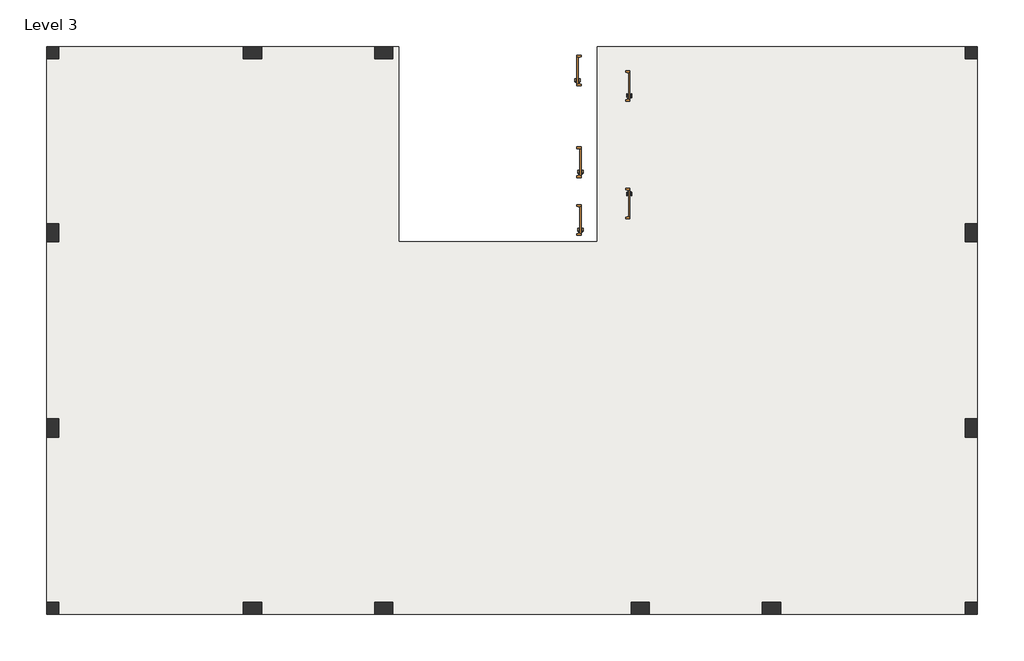
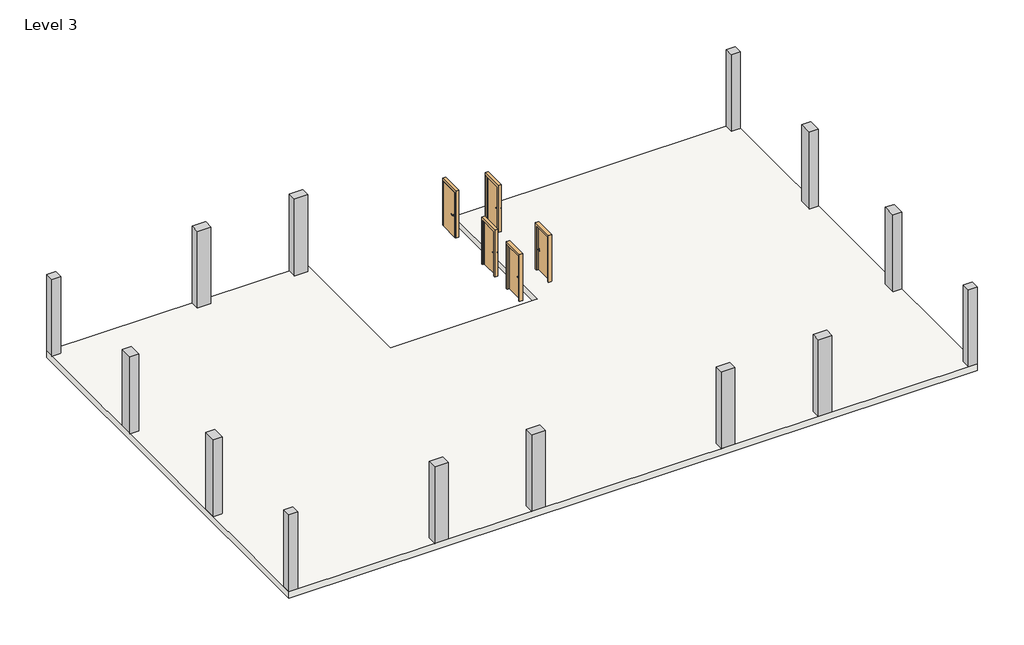
# One storey: 14 columns, 5 doors, 1 slab.
"""IFC4 building model written with IfcOpenShell, lengths in millimetres."""

import ifcopenshell
import ifcopenshell.guid

model = None  # the IFC model being written
_history = None  # IfcOwnerHistory: only IFC2X3 demands one
_inside = {}  # id of a spatial element -> (the spatial element, [elements in it])
_under = {}  # id of a project, library or spatial element -> (it, [spatial elements below it])
_declared = {}  # id of a project -> (the project, [libraries it declares])
_typed = {}  # id of a type object -> (the type object, [elements of that type])
_made_of = {}  # id of a material, layer set ... -> (it, [elements and type objects made of it])


def new_model(schema):
    """Start an empty IFC model of exactly this schema.

    Asked for "IFC4X3", IfcOpenShell would pick the latest addendum, in which some entities
    have other attributes; the version numbers below select the first issue.
    IFC2X3 requires an IfcOwnerHistory on every rooted entity: one is made here for all.
    """
    global model, _history
    if schema == "IFC4X3":
        model = ifcopenshell.file(schema_version=(4, 3, 0, 0))
    else:
        model = ifcopenshell.file(schema=schema)
    _inside.clear()
    _under.clear()
    _declared.clear()
    _typed.clear()
    _made_of.clear()
    _history = None
    if model.schema == "IFC2X3":
        org = make("IfcOrganization", Name="unknown")
        user = make(
            "IfcPersonAndOrganization",
            ThePerson=make("IfcPerson", FamilyName="unknown"),
            TheOrganization=org,
        )
        app = make(
            "IfcApplication",
            ApplicationDeveloper=org,
            Version="unknown",
            ApplicationFullName="unknown",
            ApplicationIdentifier="unknown",
        )
        _history = make(
            "IfcOwnerHistory",
            OwningUser=user,
            OwningApplication=app,
            ChangeAction="ADDED",
            CreationDate=0,
        )
    return model


def make(cls, **values):
    """One entity of the class cls with the attributes given. An attribute that is None is left unset."""
    return model.create_entity(
        cls, **{name: value for name, value in values.items() if value is not None}
    )


def rooted(cls, **values):
    """An entity with a GlobalId (a new one), such as an element, a storey or a relation."""
    return make(cls, GlobalId=ifcopenshell.guid.new(), OwnerHistory=_history, **values)


def si_unit(unit_type, name, prefix=None):
    """IfcSIUnit, for example si_unit("LENGTHUNIT", "METRE", prefix="MILLI")."""
    return make("IfcSIUnit", UnitType=unit_type, Prefix=prefix, Name=name)


def assignment(units):
    """IfcUnitAssignment: the units of a project."""
    return None if units is None else make("IfcUnitAssignment", Units=units)


def point(xyz):
    """IfcCartesianPoint."""
    return None if xyz is None else make("IfcCartesianPoint", Coordinates=xyz)


def direction(xyz):
    """IfcDirection."""
    return None if xyz is None else make("IfcDirection", DirectionRatios=xyz)


def frame(location, z_axis=None, x_axis=None):
    """IfcAxis2Placement3D, a coordinate frame: its origin and axes. An axis left out is left unset."""
    return make(
        "IfcAxis2Placement3D",
        Location=point(location),
        Axis=direction(z_axis),
        RefDirection=direction(x_axis),
    )


def frame_2d(location, x_axis=None):
    """IfcAxis2Placement2D, a coordinate frame in the plane: its origin and x axis."""
    return make(
        "IfcAxis2Placement2D", Location=point(location), RefDirection=direction(x_axis)
    )


def origin():
    """The frame at (0, 0, 0) with its axes left unset."""
    return frame((0.0, 0.0, 0.0))


def origin_with_axes():
    """The frame at (0, 0, 0) with the z axis (0, 0, 1) and the x axis (1, 0, 0) written out."""
    return frame((0.0, 0.0, 0.0), z_axis=(0.0, 0.0, 1.0), x_axis=(1.0, 0.0, 0.0))


def place(relative_to, where):
    """IfcLocalPlacement: puts the frame where relative to a parent placement (None: the world)."""
    return make(
        "IfcLocalPlacement", PlacementRelTo=relative_to, RelativePlacement=where
    )


def context(
    kind, dimensions, precision=None, world=None, true_north=None, identifier=None
):
    """IfcGeometricRepresentationContext, for example the 3D "Model" context."""
    return make(
        "IfcGeometricRepresentationContext",
        ContextIdentifier=identifier,
        ContextType=kind,
        CoordinateSpaceDimension=dimensions,
        Precision=precision,
        WorldCoordinateSystem=world,
        TrueNorth=true_north,
    )


def project(units=None, contexts=None):
    """IfcProject with its units and contexts."""
    return rooted(
        "IfcProject",
        Name="project",
        RepresentationContexts=contexts,
        UnitsInContext=assignment(units),
    )


def spatial(cls, under=None, at=None, **own):
    """A site, building, storey or space (cls), placed at a placement, below another one or the project."""
    s = rooted(cls, ObjectPlacement=at, **own)
    if under is not None:
        _under.setdefault(under.id(), (under, []))[1].append(s)
    return s


def polyline(points):
    """IfcPolyline through the points."""
    return make("IfcPolyline", Points=[point(p) for p in points])


def circle_curve(where, radius):
    """IfcCircle in the frame where."""
    return make("IfcCircle", Position=where, Radius=radius)


def ellipse_curve(where, semi_axis1, semi_axis2):
    """IfcEllipse in the frame where."""
    return make(
        "IfcEllipse", Position=where, SemiAxis1=semi_axis1, SemiAxis2=semi_axis2
    )


def trimmed(basis, trim1, trim2, sense, master):
    """IfcTrimmedCurve: the piece of a basis curve between two trims."""
    return make(
        "IfcTrimmedCurve",
        BasisCurve=basis,
        Trim1=trim1,
        Trim2=trim2,
        SenseAgreement=sense,
        MasterRepresentation=master,
    )


def segment(curve, same_sense, transition):
    """IfcCompositeCurveSegment."""
    return make(
        "IfcCompositeCurveSegment",
        Transition=transition,
        SameSense=same_sense,
        ParentCurve=curve,
    )


def composite_curve(segments, self_intersect=None):
    """IfcCompositeCurve: segments joined end to end."""
    return make("IfcCompositeCurve", Segments=segments, SelfIntersect=self_intersect)


def outline(outer, holes=None, kind="AREA"):
    """IfcArbitraryClosedProfileDef: a profile drawn as a closed curve; with holes, ...WithVoids."""
    if holes is None:
        return make("IfcArbitraryClosedProfileDef", ProfileType=kind, OuterCurve=outer)
    return make(
        "IfcArbitraryProfileDefWithVoids",
        ProfileType=kind,
        OuterCurve=outer,
        InnerCurves=holes,
    )


def extrude(swept, where, along, depth):
    """IfcExtrudedAreaSolid: the profile swept, set in the frame where, extruded along a direction by depth."""
    return make(
        "IfcExtrudedAreaSolid",
        SweptArea=swept,
        Position=where,
        ExtrudedDirection=direction(along),
        Depth=depth,
    )


def faces_of(points, faces, orient=None, outer=None):
    """IfcFace entities. A face is a list of loops; a loop is a list of indices into points, from 0.

    orient and outer hold one flag for each loop. By default every Orientation is true, the
    first loop of a face is its IfcFaceOuterBound and the others are IfcFaceBound.
    """
    made = []
    for i, loops in enumerate(faces):
        bounds = []
        for j, loop in enumerate(loops):
            is_outer = j == 0 if outer is None else outer[i][j]
            bounds.append(
                make(
                    "IfcFaceOuterBound" if is_outer else "IfcFaceBound",
                    Bound=make("IfcPolyLoop", Polygon=[points[k] for k in loop]),
                    Orientation=True if orient is None else orient[i][j],
                )
            )
        made.append(make("IfcFace", Bounds=bounds))
    return made


def faceted_brep(points, faces, orient=None, outer=None, voids=None):
    """IfcFacetedBrep: a solid bounded by flat faces; with voids (closed shells), ...WithVoids."""
    shared = [point(p) for p in points]
    hull = make("IfcClosedShell", CfsFaces=faces_of(shared, faces, orient, outer))
    if voids is None:
        return make("IfcFacetedBrep", Outer=hull)
    return make(
        "IfcFacetedBrepWithVoids",
        Outer=hull,
        Voids=[
            make(cls, CfsFaces=faces_of(shared, fs, o, b)) for cls, fs, o, b in voids
        ],
    )


def shape(context_of_items, identifier, shape_type, items):
    """IfcShapeRepresentation: the items that make up one representation, for example the "Body"."""
    return make(
        "IfcShapeRepresentation",
        ContextOfItems=context_of_items,
        RepresentationIdentifier=identifier,
        RepresentationType=shape_type,
        Items=items,
    )


def source(mapping_origin, context_of_items, identifier, shape_type, items):
    """IfcRepresentationMap: a shape defined once, which mapped items show again and again."""
    return make(
        "IfcRepresentationMap",
        MappingOrigin=mapping_origin,
        MappedRepresentation=shape(context_of_items, identifier, shape_type, items),
    )


def transform(
    local_origin,
    x_axis=None,
    y_axis=None,
    z_axis=None,
    scale=None,
    scale2=None,
    scale3=None,
    uniform=True,
):
    """IfcCartesianTransformationOperator3D, or its non-uniform kind. x_axis, y_axis, z_axis: its Axis1, 2, 3."""
    if uniform:
        return make(
            "IfcCartesianTransformationOperator3D",
            Axis1=direction(x_axis),
            Axis2=direction(y_axis),
            LocalOrigin=point(local_origin),
            Scale=scale,
            Axis3=direction(z_axis),
        )
    return make(
        "IfcCartesianTransformationOperator3DnonUniform",
        Axis1=direction(x_axis),
        Axis2=direction(y_axis),
        LocalOrigin=point(local_origin),
        Scale=scale,
        Axis3=direction(z_axis),
        Scale2=scale2,
        Scale3=scale3,
    )


def mapped(mapping_source, mapping_target):
    """IfcMappedItem: shows the shape of a source again, moved by a transform."""
    return make(
        "IfcMappedItem", MappingSource=mapping_source, MappingTarget=mapping_target
    )


def made_of(thing, what):
    """Note that an element or type object is made of a material, layer set ...; save() writes the relation."""
    if what is not None:
        _made_of.setdefault(what.id(), (what, []))[1].append(thing)
    return thing


def element(
    cls,
    number,
    at=None,
    inside=None,
    cuts=None,
    type_object=None,
    material=None,
    context=None,
    identifier="Body",
    shape_type=None,
    held_by="IfcProductDefinitionShape",
    body=None,
    shapes=None,
    **own,
):
    """One element of the class cls, such as IfcWall. Its Tag is "e" and its number.

    at: its placement. inside: the storey or other place that contains it. cuts: it is an
    opening in that element (IfcRelVoidsElement). A single representation is given by context,
    identifier, shape_type and body (its items); several are given by shapes. held_by: the class
    of the entity that holds the representations. save() writes the other relations.
    """
    e = rooted(cls, Tag="e%d" % number, ObjectPlacement=at, **own)
    if body is not None:
        shapes = [shape(context, identifier, shape_type, body)]
    if shapes is not None:
        e.Representation = make(held_by, Representations=shapes)
    if inside is not None:
        _inside.setdefault(inside.id(), (inside, []))[1].append(e)
    if cuts is not None:
        rooted(
            "IfcRelVoidsElement", RelatingBuildingElement=cuts, RelatedOpeningElement=e
        )
    if type_object is not None:
        _typed.setdefault(type_object.id(), (type_object, []))[1].append(e)
    return made_of(e, material)


def aggregate(whole, parts):
    """IfcRelAggregates: a whole, such as a stair, and the parts it consists of."""
    return rooted("IfcRelAggregates", RelatingObject=whole, RelatedObjects=parts)


def save(model, path):
    """Write the relations noted so far, then the file.

    IfcRelAggregates (storeys below a building ...), IfcRelContainedInSpatialStructure (elements
    in a storey), IfcRelDefinesByType, IfcRelAssociatesMaterial and IfcRelDeclares: one each for
    every whole, place, type object, material and project.
    """
    for whole, parts in _under.values():
        aggregate(whole, parts)
    for where, things in _inside.values():
        rooted(
            "IfcRelContainedInSpatialStructure",
            RelatedElements=things,
            RelatingStructure=where,
        )
    for kind, things in _typed.values():
        rooted("IfcRelDefinesByType", RelatedObjects=things, RelatingType=kind)
    for what, things in _made_of.values():
        rooted("IfcRelAssociatesMaterial", RelatedObjects=things, RelatingMaterial=what)
    for by, libraries in _declared.values():
        rooted("IfcRelDeclares", RelatingContext=by, RelatedDefinitions=libraries)
    model.write(path)


def plane_surface(at):
    """IfcPlane: the flat surface through the origin of the frame at, square to its z axis."""
    return make("IfcPlane", Position=at)


def cylinder_surface(at, radius):
    """IfcCylindricalSurface: all points at the distance radius from the z axis of the frame at."""
    return make("IfcCylindricalSurface", Position=at, Radius=radius)


def revolved_surface(curve, axis_point, axis_direction):
    """IfcSurfaceOfRevolution: the curve turned about the line through axis_point along axis_direction."""
    return make(
        "IfcSurfaceOfRevolution",
        SweptCurve=make("IfcArbitraryOpenProfileDef", ProfileType="CURVE", Curve=curve),
        AxisPosition=make("IfcAxis1Placement", Location=point(axis_point), Axis=direction(axis_direction)),
    )


def advanced_brep(points, edges, surfaces, faces):
    """IfcAdvancedBrep: a solid bounded by faces that lie on surfaces and meet in shared edges.

    An edge is (start, end): straight between two places in points (the first is 0);
    or (start, end, curve); or (start, end, curve, False) where it runs against its curve.
    A face is (place in surfaces, loops), or (place, loops, False) where it looks against
    its surface's normal. A loop lists edges by number (the first is 1), with a minus sign
    where the edge is run from its end to its start. The first loop is the outer one.
    """
    corners = [point(p) for p in points]
    vertices = [make("IfcVertexPoint", VertexGeometry=c) for c in corners]
    made = []
    for start, end, *more in edges:
        made.append(
            make(
                "IfcEdgeCurve",
                EdgeStart=vertices[start],
                EdgeEnd=vertices[end],
                EdgeGeometry=more[0] if more else make("IfcPolyline", Points=[corners[start], corners[end]]),
                SameSense=more[1] if len(more) > 1 else True,
            )
        )
    hull = []
    for where, loops, *sense in faces:
        bounds = []
        for j, loop in enumerate(loops):
            ring = [make("IfcOrientedEdge", EdgeElement=made[abs(k) - 1], Orientation=k > 0) for k in loop]
            bounds.append(
                make(
                    "IfcFaceOuterBound" if j == 0 else "IfcFaceBound",
                    Bound=make("IfcEdgeLoop", EdgeList=ring),
                    Orientation=True,
                )
            )
        hull.append(make("IfcAdvancedFace", Bounds=bounds, FaceSurface=surfaces[where], SameSense=sense[0] if sense else True))
    return make("IfcAdvancedBrep", Outer=make("IfcClosedShell", CfsFaces=hull))


def door_9f6fe377(model_context):
    return source(origin(), model_context, "Body", "SolidModel", [
        advanced_brep(
        [(-392.190625, -25.3375, 1016.0), (-372.190625, -25.3375, 1016.0), (-392.190625, 4.6625, 1016.0), (-372.190625, 4.6625, 1016.0), (-367.190625, 9.6625, 1016.0), (-367.190625, 29.6625, 1016.0), (-262.190625, 29.6625, 1016.0), (-262.190625, 9.6625, 1016.0)],
        [
            (0, 1, circle_curve(frame((-382.190625, -25.3375, 1016.0), z_axis=(0.0, -1.0, 0.0), x_axis=(1.0, 0.0, 0.0)), 10.0)),
            (1, 0, circle_curve(frame((-382.190625, -25.3375, 1016.0), z_axis=(0.0, -1.0, 0.0), x_axis=(1.0, 0.0, 0.0)), 10.0)),
            (0, 2),
            (2, 3, circle_curve(frame((-382.190625, 4.6625, 1016.0), z_axis=(0.0, -1.0, 0.0), x_axis=(1.0, 0.0, 0.0)), 10.0)),
            (3, 1),
            (3, 2, circle_curve(frame((-382.190625, 4.6625, 1016.0), z_axis=(0.0, -1.0, 0.0), x_axis=(1.0, 0.0, 0.0)), 10.0)),
            (4, 3, circle_curve(frame((-367.190625, 4.6625, 1016.0), z_axis=(0.0, 0.0, 1.0), x_axis=(-1.0, 0.0, 0.0)), 5.0)),
            (2, 5, circle_curve(frame((-367.190625, 4.6625, 1016.0), z_axis=(0.0, 0.0, -1.0), x_axis=(-1.0, 0.0, 0.0)), 25.0)),
            (5, 4, circle_curve(frame((-367.190625, 19.6625, 1016.0), z_axis=(-1.0, 0.0, 0.0), x_axis=(0.0, -1.0, 0.0)), 10.0)),
            (4, 5, circle_curve(frame((-367.190625, 19.6625, 1016.0), z_axis=(-1.0, 0.0, 0.0), x_axis=(0.0, -1.0, 0.0)), 10.0)),
            (6, 7, circle_curve(frame((-262.190625, 19.6625, 1016.0), z_axis=(1.0, 0.0, 0.0), x_axis=(0.0, -1.0, 0.0)), 10.0)),
            (7, 6, circle_curve(frame((-262.190625, 19.6625, 1016.0), z_axis=(1.0, 0.0, 0.0), x_axis=(0.0, -1.0, 0.0)), 10.0)),
            (5, 6),
            (7, 4),
        ],
        [
            plane_surface(frame((-382.190625, -25.3375, 1016.0), z_axis=(0.0, -1.0, 0.0), x_axis=(0.0, 0.0, 1.0))),
            cylinder_surface(frame((-382.190625, -25.3375, 1016.0), z_axis=(0.0, -1.0, 0.0), x_axis=(1.0, 0.0, 0.0)), 10.0),
            revolved_surface(trimmed(ellipse_curve(frame((-382.190625, 4.6625, 1016.0), z_axis=(0.0, -1.0, 0.0), x_axis=(1.0, 0.0, 0.0)), 10.0, 10.0), [point((-392.190625, 4.6625, 1016.0))], [point((-372.190625, 4.6625, 1016.0))], True, "CARTESIAN"), (-367.190625, 4.6625, 1016.0), (0.0, 0.0, -1.0)),
            revolved_surface(trimmed(ellipse_curve(frame((-382.190625, 4.6625, 1016.0), z_axis=(0.0, -1.0, 0.0), x_axis=(1.0, 0.0, 0.0)), 10.0, 10.0), [point((-372.190625, 4.6625, 1016.0))], [point((-392.190625, 4.6625, 1016.0))], True, "CARTESIAN"), (-367.190625, 4.6625, 1016.0), (0.0, 0.0, -1.0)),
            plane_surface(frame((-262.190625, 19.6625, 1016.0), z_axis=(1.0, 0.0, 0.0), x_axis=(0.0, 0.0, 1.0))),
            cylinder_surface(frame((-367.190625, 19.6625, 1016.0), z_axis=(-1.0, 0.0, 0.0), x_axis=(0.0, -1.0, 0.0)), 10.0),
        ],
        [
            (0, [[1, 2]]),
            (1, [[-1, 3, 4, 5]]),
            (1, [[-2, -5, 6, -3]]),
            (2, [[7, -4, 8, 9]]),
            (3, [[-8, -6, -7, 10]]),
            (4, [[11, 12]]),
            (5, [[-9, 13, -12, 14]]),
            (5, [[-10, -14, -11, -13]]),
        ],
    ),
        extrude(outline(composite_curve([segment(trimmed(circle_curve(frame_2d((1016.0, -384.690625)), 30.0), [point((1016.0, -414.690625))], [point((1016.0, -354.690625))], False, "CARTESIAN"), True, "CONTINUOUS"), segment(trimmed(circle_curve(frame_2d((1016.0, -384.690625)), 30.0), [point((1016.0, -354.690625))], [point((1016.0, -414.690625))], False, "CARTESIAN"), True, "CONTINUOUS")], self_intersect=False)), frame((0.0, -33.3375, 0.0), z_axis=(0.0, 1.0, 0.0), x_axis=(0.0, 0.0, 1.0)), (0.0, 0.0, 1.0), 8.0),
        advanced_brep(
        [(-392.190625, -85.7875, 1016.0), (-372.190625, -85.7875, 1016.0), (-372.190625, -115.7875, 1016.0), (-392.190625, -115.7875, 1016.0), (-367.190625, -120.7875, 1016.0), (-367.190625, -140.7875, 1016.0), (-262.190625, -140.7875, 1016.0), (-262.190625, -120.7875, 1016.0)],
        [
            (0, 1, circle_curve(frame((-382.190625, -85.7875, 1016.0), z_axis=(0.0, 1.0, 0.0), x_axis=(1.0, 0.0, 0.0)), 10.0)),
            (1, 0, circle_curve(frame((-382.190625, -85.7875, 1016.0), z_axis=(0.0, 1.0, 0.0), x_axis=(1.0, 0.0, 0.0)), 10.0)),
            (1, 2),
            (2, 3, circle_curve(frame((-382.190625, -115.7875, 1016.0), z_axis=(0.0, 1.0, 0.0), x_axis=(1.0, 0.0, 0.0)), 10.0)),
            (3, 0),
            (3, 2, circle_curve(frame((-382.190625, -115.7875, 1016.0), z_axis=(0.0, 1.0, 0.0), x_axis=(1.0, 0.0, 0.0)), 10.0)),
            (4, 5, circle_curve(frame((-367.190625, -130.7875, 1016.0), z_axis=(-1.0, 0.0, 0.0), x_axis=(0.0, 1.0, 0.0)), 10.0)),
            (5, 3, circle_curve(frame((-367.190625, -115.7875, 1016.0), z_axis=(0.0, 0.0, -1.0), x_axis=(-1.0, 0.0, 0.0)), 25.0)),
            (2, 4, circle_curve(frame((-367.190625, -115.7875, 1016.0), z_axis=(0.0, 0.0, 1.0), x_axis=(-1.0, 0.0, 0.0)), 5.0)),
            (5, 4, circle_curve(frame((-367.190625, -130.7875, 1016.0), z_axis=(-1.0, 0.0, 0.0), x_axis=(0.0, 1.0, 0.0)), 10.0)),
            (6, 7, circle_curve(frame((-262.190625, -130.7875, 1016.0), z_axis=(1.0, 0.0, 0.0), x_axis=(0.0, 1.0, 0.0)), 10.0)),
            (7, 6, circle_curve(frame((-262.190625, -130.7875, 1016.0), z_axis=(1.0, 0.0, 0.0), x_axis=(0.0, 1.0, 0.0)), 10.0)),
            (4, 7),
            (6, 5),
        ],
        [
            plane_surface(frame((-382.190625, -85.7875, 1016.0), z_axis=(0.0, 1.0, 0.0), x_axis=(0.0, 0.0, 1.0))),
            cylinder_surface(frame((-382.190625, -85.7875, 1016.0), z_axis=(0.0, 1.0, 0.0), x_axis=(1.0, 0.0, 0.0)), 10.0),
            revolved_surface(trimmed(ellipse_curve(frame((-382.190625, -115.7875, 1016.0), z_axis=(0.0, -1.0, 0.0), x_axis=(1.0, 0.0, 0.0)), 10.0, 10.0), [point((-392.190625, -115.7875, 1016.0))], [point((-372.190625, -115.7875, 1016.0))], True, "CARTESIAN"), (-367.190625, -115.7875, 1016.0), (0.0, 0.0, -1.0)),
            revolved_surface(trimmed(ellipse_curve(frame((-382.190625, -115.7875, 1016.0), z_axis=(0.0, -1.0, 0.0), x_axis=(1.0, 0.0, 0.0)), 10.0, 10.0), [point((-372.190625, -115.7875, 1016.0))], [point((-392.190625, -115.7875, 1016.0))], True, "CARTESIAN"), (-367.190625, -115.7875, 1016.0), (0.0, 0.0, -1.0)),
            plane_surface(frame((-262.190625, -130.7875, 1016.0), z_axis=(1.0, 0.0, 0.0), x_axis=(0.0, 0.0, 1.0))),
            cylinder_surface(frame((-367.190625, -130.7875, 1016.0), z_axis=(-1.0, 0.0, 0.0), x_axis=(0.0, 1.0, 0.0)), 10.0),
        ],
        [
            (0, [[1, 2]]),
            (1, [[3, 4, 5, -2]]),
            (1, [[-5, 6, -3, -1]]),
            (2, [[7, 8, -4, 9]]),
            (3, [[10, -9, -6, -8]]),
            (4, [[11, 12]]),
            (5, [[13, -11, 14, -7]]),
            (5, [[-14, -12, -13, -10]]),
        ],
    ),
        extrude(outline(composite_curve([segment(trimmed(circle_curve(frame_2d((1016.0, -384.690625)), 30.0), [point((1016.0, -414.690625))], [point((1016.0, -354.690625))], False, "CARTESIAN"), True, "CONTINUOUS"), segment(trimmed(circle_curve(frame_2d((1016.0, -384.690625)), 30.0), [point((1016.0, -354.690625))], [point((1016.0, -414.690625))], False, "CARTESIAN"), True, "CONTINUOUS")], self_intersect=False)), frame((0.0, -85.7875, 0.0), z_axis=(0.0, 1.0, 0.0), x_axis=(0.0, 0.0, 1.0)), (0.0, 0.0, 1.0), 8.0),
        faceted_brep([(457.2, -28.575, 0.0), (441.325, -28.575, 0.0), (441.325, 19.05, 0.0), (457.2, 19.05, 0.0), (457.2, 68.2625, 0.0), (508.0, 68.2625, 0.0), (508.0, -77.7875, 0.0), (457.2, -77.7875, 0.0), (457.2, -77.7875, 2133.6), (457.2, -28.575, 2133.6), (508.0, -77.7875, 2235.2), (-508.0, -77.7875, 2235.2), (-508.0, -77.7875, 0.0), (-457.2, -77.7875, 0.0), (-457.2, -77.7875, 2133.6), (508.0, 68.2625, 2235.2), (457.2, 68.2625, 2133.6), (-457.2, 68.2625, 2133.6), (-457.2, 68.2625, 0.0), (-508.0, 68.2625, 0.0), (-508.0, 68.2625, 2235.2), (457.2, 19.05, 2133.6), (441.325, 19.05, 2117.725), (-441.325, 19.05, 2117.725), (-441.325, 19.05, 0.0), (-457.2, 19.05, 0.0), (-457.2, 19.05, 2133.6), (441.325, -28.575, 2117.725), (-457.2, -28.575, 2133.6), (-457.2, -28.575, 0.0), (-441.325, -28.575, 0.0), (-441.325, -28.575, 2117.725)], [[[0, 1, 2, 3, 4, 5, 6, 7]], [[7, 8, 9, 0]], [[6, 10, 11, 12, 13, 14, 8, 7]], [[5, 15, 10, 6]], [[4, 16, 17, 18, 19, 20, 15, 5]], [[3, 21, 16, 4]], [[2, 22, 23, 24, 25, 26, 21, 3]], [[1, 27, 22, 2]], [[0, 9, 28, 29, 30, 31, 27, 1]], [[8, 14, 28, 9]], [[16, 21, 26, 17]], [[22, 27, 31, 23]], [[12, 19, 18, 25, 24, 30, 29, 13]], [[13, 29, 28, 14]], [[11, 20, 19, 12]], [[17, 26, 25, 18]], [[23, 31, 30, 24]], [[15, 20, 11, 10]]]),
        extrude(outline(polyline([(457.2, -33.3375), (457.2, -77.7875), (-457.2, -77.7875), (-457.2, -33.3375), (457.2, -33.3375)])), origin_with_axes(), (0.0, 0.0, 1.0), 2133.6),
    ])


def door_87fe937e(model_context):
    return source(origin(), model_context, "Body", "SolidModel", [
        advanced_brep(
        [(-392.190625, 25.3375, 1016.0), (-372.190625, 25.3375, 1016.0), (-372.190625, -4.6625, 1016.0), (-392.190625, -4.6625, 1016.0), (-367.190625, -9.6625, 1016.0), (-367.190625, -29.6625, 1016.0), (-262.190625, -29.6625, 1016.0), (-262.190625, -9.6625, 1016.0)],
        [
            (0, 1, circle_curve(frame((-382.190625, 25.3375, 1016.0), z_axis=(0.0, 1.0, 0.0), x_axis=(1.0, 0.0, 0.0)), 10.0)),
            (1, 0, circle_curve(frame((-382.190625, 25.3375, 1016.0), z_axis=(0.0, 1.0, 0.0), x_axis=(1.0, 0.0, 0.0)), 10.0)),
            (1, 2),
            (2, 3, circle_curve(frame((-382.190625, -4.6625, 1016.0), z_axis=(0.0, 1.0, 0.0), x_axis=(1.0, 0.0, 0.0)), 10.0)),
            (3, 0),
            (3, 2, circle_curve(frame((-382.190625, -4.6625, 1016.0), z_axis=(0.0, 1.0, 0.0), x_axis=(1.0, 0.0, 0.0)), 10.0)),
            (4, 5, circle_curve(frame((-367.190625, -19.6625, 1016.0), z_axis=(-1.0, 0.0, 0.0), x_axis=(0.0, 1.0, 0.0)), 10.0)),
            (5, 3, circle_curve(frame((-367.190625, -4.6625, 1016.0), z_axis=(0.0, 0.0, -1.0), x_axis=(-1.0, 0.0, 0.0)), 25.0)),
            (2, 4, circle_curve(frame((-367.190625, -4.6625, 1016.0), z_axis=(0.0, 0.0, 1.0), x_axis=(-1.0, 0.0, 0.0)), 5.0)),
            (5, 4, circle_curve(frame((-367.190625, -19.6625, 1016.0), z_axis=(-1.0, 0.0, 0.0), x_axis=(0.0, 1.0, 0.0)), 10.0)),
            (6, 7, circle_curve(frame((-262.190625, -19.6625, 1016.0), z_axis=(1.0, 0.0, 0.0), x_axis=(0.0, 1.0, 0.0)), 10.0)),
            (7, 6, circle_curve(frame((-262.190625, -19.6625, 1016.0), z_axis=(1.0, 0.0, 0.0), x_axis=(0.0, 1.0, 0.0)), 10.0)),
            (4, 7),
            (6, 5),
        ],
        [
            plane_surface(frame((-382.190625, 25.3375, 1016.0), z_axis=(0.0, 1.0, 0.0), x_axis=(0.0, 0.0, 1.0))),
            cylinder_surface(frame((-382.190625, 25.3375, 1016.0), z_axis=(0.0, 1.0, 0.0), x_axis=(1.0, 0.0, 0.0)), 10.0),
            revolved_surface(trimmed(ellipse_curve(frame((-382.190625, -4.6625, 1016.0), z_axis=(0.0, -1.0, 0.0), x_axis=(1.0, 0.0, 0.0)), 10.0, 10.0), [point((-392.190625, -4.6625, 1016.0))], [point((-372.190625, -4.6625, 1016.0))], True, "CARTESIAN"), (-367.190625, -4.6625, 1016.0), (0.0, 0.0, -1.0)),
            revolved_surface(trimmed(ellipse_curve(frame((-382.190625, -4.6625, 1016.0), z_axis=(0.0, -1.0, 0.0), x_axis=(1.0, 0.0, 0.0)), 10.0, 10.0), [point((-372.190625, -4.6625, 1016.0))], [point((-392.190625, -4.6625, 1016.0))], True, "CARTESIAN"), (-367.190625, -4.6625, 1016.0), (0.0, 0.0, -1.0)),
            plane_surface(frame((-262.190625, -19.6625, 1016.0), z_axis=(1.0, 0.0, 0.0), x_axis=(0.0, 0.0, 1.0))),
            cylinder_surface(frame((-367.190625, -19.6625, 1016.0), z_axis=(-1.0, 0.0, 0.0), x_axis=(0.0, 1.0, 0.0)), 10.0),
        ],
        [
            (0, [[1, 2]]),
            (1, [[3, 4, 5, -2]]),
            (1, [[-5, 6, -3, -1]]),
            (2, [[7, 8, -4, 9]]),
            (3, [[10, -9, -6, -8]]),
            (4, [[11, 12]]),
            (5, [[13, -11, 14, -7]]),
            (5, [[-14, -12, -13, -10]]),
        ],
    ),
        extrude(outline(composite_curve([segment(trimmed(circle_curve(frame_2d((1016.0, -384.690625)), 30.0), [point((1016.0, -414.690625))], [point((1016.0, -354.690625))], False, "CARTESIAN"), True, "CONTINUOUS"), segment(trimmed(circle_curve(frame_2d((1016.0, -384.690625)), 30.0), [point((1016.0, -354.690625))], [point((1016.0, -414.690625))], False, "CARTESIAN"), True, "CONTINUOUS")], self_intersect=False)), frame((0.0, 25.3375, 0.0), z_axis=(0.0, 1.0, 0.0), x_axis=(0.0, 0.0, 1.0)), (0.0, 0.0, 1.0), 8.0),
        advanced_brep(
        [(-392.190625, 85.7875, 1016.0), (-372.190625, 85.7875, 1016.0), (-392.190625, 115.7875, 1016.0), (-372.190625, 115.7875, 1016.0), (-367.190625, 120.7875, 1016.0), (-367.190625, 140.7875, 1016.0), (-262.190625, 140.7875, 1016.0), (-262.190625, 120.7875, 1016.0)],
        [
            (0, 1, circle_curve(frame((-382.190625, 85.7875, 1016.0), z_axis=(0.0, -1.0, 0.0), x_axis=(1.0, 0.0, 0.0)), 10.0)),
            (1, 0, circle_curve(frame((-382.190625, 85.7875, 1016.0), z_axis=(0.0, -1.0, 0.0), x_axis=(1.0, 0.0, 0.0)), 10.0)),
            (0, 2),
            (2, 3, circle_curve(frame((-382.190625, 115.7875, 1016.0), z_axis=(0.0, -1.0, 0.0), x_axis=(1.0, 0.0, 0.0)), 10.0)),
            (3, 1),
            (3, 2, circle_curve(frame((-382.190625, 115.7875, 1016.0), z_axis=(0.0, -1.0, 0.0), x_axis=(1.0, 0.0, 0.0)), 10.0)),
            (4, 3, circle_curve(frame((-367.190625, 115.7875, 1016.0), z_axis=(0.0, 0.0, 1.0), x_axis=(-1.0, 0.0, 0.0)), 5.0)),
            (2, 5, circle_curve(frame((-367.190625, 115.7875, 1016.0), z_axis=(0.0, 0.0, -1.0), x_axis=(-1.0, 0.0, 0.0)), 25.0)),
            (5, 4, circle_curve(frame((-367.190625, 130.7875, 1016.0), z_axis=(-1.0, 0.0, 0.0), x_axis=(0.0, -1.0, 0.0)), 10.0)),
            (4, 5, circle_curve(frame((-367.190625, 130.7875, 1016.0), z_axis=(-1.0, 0.0, 0.0), x_axis=(0.0, -1.0, 0.0)), 10.0)),
            (6, 7, circle_curve(frame((-262.190625, 130.7875, 1016.0), z_axis=(1.0, 0.0, 0.0), x_axis=(0.0, -1.0, 0.0)), 10.0)),
            (7, 6, circle_curve(frame((-262.190625, 130.7875, 1016.0), z_axis=(1.0, 0.0, 0.0), x_axis=(0.0, -1.0, 0.0)), 10.0)),
            (5, 6),
            (7, 4),
        ],
        [
            plane_surface(frame((-382.190625, 85.7875, 1016.0), z_axis=(0.0, -1.0, 0.0), x_axis=(0.0, 0.0, 1.0))),
            cylinder_surface(frame((-382.190625, 85.7875, 1016.0), z_axis=(0.0, -1.0, 0.0), x_axis=(1.0, 0.0, 0.0)), 10.0),
            revolved_surface(trimmed(ellipse_curve(frame((-382.190625, 115.7875, 1016.0), z_axis=(0.0, -1.0, 0.0), x_axis=(1.0, 0.0, 0.0)), 10.0, 10.0), [point((-392.190625, 115.7875, 1016.0))], [point((-372.190625, 115.7875, 1016.0))], True, "CARTESIAN"), (-367.190625, 115.7875, 1016.0), (0.0, 0.0, -1.0)),
            revolved_surface(trimmed(ellipse_curve(frame((-382.190625, 115.7875, 1016.0), z_axis=(0.0, -1.0, 0.0), x_axis=(1.0, 0.0, 0.0)), 10.0, 10.0), [point((-372.190625, 115.7875, 1016.0))], [point((-392.190625, 115.7875, 1016.0))], True, "CARTESIAN"), (-367.190625, 115.7875, 1016.0), (0.0, 0.0, -1.0)),
            plane_surface(frame((-262.190625, 130.7875, 1016.0), z_axis=(1.0, 0.0, 0.0), x_axis=(0.0, 0.0, 1.0))),
            cylinder_surface(frame((-367.190625, 130.7875, 1016.0), z_axis=(-1.0, 0.0, 0.0), x_axis=(0.0, -1.0, 0.0)), 10.0),
        ],
        [
            (0, [[1, 2]]),
            (1, [[-1, 3, 4, 5]]),
            (1, [[-2, -5, 6, -3]]),
            (2, [[7, -4, 8, 9]]),
            (3, [[-8, -6, -7, 10]]),
            (4, [[11, 12]]),
            (5, [[-9, 13, -12, 14]]),
            (5, [[-10, -14, -11, -13]]),
        ],
    ),
        extrude(outline(composite_curve([segment(trimmed(circle_curve(frame_2d((1016.0, -384.690625)), 30.0), [point((1016.0, -414.690625))], [point((1016.0, -354.690625))], False, "CARTESIAN"), True, "CONTINUOUS"), segment(trimmed(circle_curve(frame_2d((1016.0, -384.690625)), 30.0), [point((1016.0, -354.690625))], [point((1016.0, -414.690625))], False, "CARTESIAN"), True, "CONTINUOUS")], self_intersect=False)), frame((0.0, 77.7875, 0.0), z_axis=(0.0, 1.0, 0.0), x_axis=(0.0, 0.0, 1.0)), (0.0, 0.0, 1.0), 8.0),
        faceted_brep([(457.2, 28.575, 0.0), (457.2, 77.7875, 0.0), (508.0, 77.7875, 0.0), (508.0, -68.2625, 0.0), (457.2, -68.2625, 0.0), (457.2, -19.05, 0.0), (441.325, -19.05, 0.0), (441.325, 28.575, 0.0), (457.2, 28.575, 2133.6), (457.2, 77.7875, 2133.6), (-457.2, 77.7875, 2133.6), (-457.2, 77.7875, 0.0), (-508.0, 77.7875, 0.0), (-508.0, 77.7875, 2235.2), (508.0, 77.7875, 2235.2), (508.0, -68.2625, 2235.2), (-508.0, -68.2625, 2235.2), (-508.0, -68.2625, 0.0), (-457.2, -68.2625, 0.0), (-457.2, -68.2625, 2133.6), (457.2, -68.2625, 2133.6), (457.2, -19.05, 2133.6), (-457.2, -19.05, 2133.6), (-457.2, -19.05, 0.0), (-441.325, -19.05, 0.0), (-441.325, -19.05, 2117.725), (441.325, -19.05, 2117.725), (441.325, 28.575, 2117.725), (-441.325, 28.575, 2117.725), (-441.325, 28.575, 0.0), (-457.2, 28.575, 0.0), (-457.2, 28.575, 2133.6)], [[[0, 1, 2, 3, 4, 5, 6, 7]], [[1, 0, 8, 9]], [[2, 1, 9, 10, 11, 12, 13, 14]], [[3, 2, 14, 15]], [[4, 3, 15, 16, 17, 18, 19, 20]], [[5, 4, 20, 21]], [[6, 5, 21, 22, 23, 24, 25, 26]], [[7, 6, 26, 27]], [[0, 7, 27, 28, 29, 30, 31, 8]], [[9, 8, 31, 10]], [[20, 19, 22, 21]], [[26, 25, 28, 27]], [[12, 11, 30, 29, 24, 23, 18, 17]], [[11, 10, 31, 30]], [[13, 12, 17, 16]], [[19, 18, 23, 22]], [[25, 24, 29, 28]], [[15, 14, 13, 16]]]),
        extrude(outline(polyline([(457.2, 33.3375), (-457.2, 33.3375), (-457.2, 77.7875), (457.2, 77.7875), (457.2, 33.3375)])), origin_with_axes(), (0.0, 0.0, 1.0), 2133.6),
    ])


model = new_model("IFC4")

# Units and contexts
model_context = context("Model", 3, world=origin())
ifc_project = project(units=[si_unit("LENGTHUNIT", "METRE", prefix="MILLI")], contexts=[model_context])

# Site, building, storey
site = spatial("IfcSite", under=ifc_project)
building = spatial("IfcBuilding", under=site)
storey = spatial("IfcBuildingStorey", under=building, Name="Level 3", Elevation=7315.2)

# Columns
placement = place(None, origin())
element("IfcColumn", 1, ObjectType="Rectangular Column : 24\" x 24\"", at=placement, inside=storey, context=model_context, shape_type="SweptSolid", body=[
    extrude(outline(polyline([(-16253.4122732, 9291.5015304), (-16253.4122732, 8885.1015304), (-16659.8122732, 8885.1015304), (-16659.8122732, 9291.5015304), (-16253.4122732, 9291.5015304)])), frame((0.0, 0.0, 7315.2), z_axis=(0.0, 0.0, 1.0), x_axis=(1.0, 0.0, 0.0)), (0.0, 0.0, 1.0), 3657.6),
])
element("IfcColumn", 2, ObjectType="Rectangular Column : 24\" x 24\"", at=placement, inside=storey, context=model_context, shape_type="SweptSolid", body=[
    extrude(outline(polyline([(-16253.4122732, 3398.7015304), (-16253.4122732, 2789.1015304), (-16659.8122732, 2789.1015304), (-16659.8122732, 3398.7015304), (-16253.4122732, 3398.7015304)])), frame((0.0, 0.0, 7315.2), z_axis=(0.0, 0.0, 1.0), x_axis=(1.0, 0.0, 0.0)), (0.0, 0.0, 1.0), 3657.6),
])
element("IfcColumn", 3, ObjectType="Rectangular Column : 24\" x 24\"", at=placement, inside=storey, context=model_context, shape_type="SweptSolid", body=[
    extrude(outline(polyline([(-9497.0122732, 8885.1015304), (-10106.6122732, 8885.1015304), (-10106.6122732, 9291.5015304), (-9497.0122732, 9291.5015304), (-9497.0122732, 8885.1015304)])), frame((0.0, 0.0, 7315.2), z_axis=(0.0, 0.0, 1.0), x_axis=(1.0, 0.0, 0.0)), (0.0, 0.0, 1.0), 3657.6),
])
element("IfcColumn", 4, ObjectType="Rectangular Column : 24\" x 24\"", at=placement, inside=storey, context=model_context, shape_type="SweptSolid", body=[
    extrude(outline(polyline([(-5128.2122732, 8885.1015304), (-5737.8122732, 8885.1015304), (-5737.8122732, 9291.5015304), (-5128.2122732, 9291.5015304), (-5128.2122732, 8885.1015304)])), frame((0.0, 0.0, 7315.2), z_axis=(0.0, 0.0, 1.0), x_axis=(1.0, 0.0, 0.0)), (0.0, 0.0, 1.0), 3657.6),
])
element("IfcColumn", 5, ObjectType="Rectangular Column : 24\" x 24\"", at=placement, inside=storey, context=model_context, shape_type="SweptSolid", body=[
    extrude(outline(polyline([(14328.1877268, 8885.1015304), (13921.7877268, 8885.1015304), (13921.7877268, 9291.5015304), (14328.1877268, 9291.5015304), (14328.1877268, 8885.1015304)])), frame((0.0, 0.0, 7315.2), z_axis=(0.0, 0.0, 1.0), x_axis=(1.0, 0.0, 0.0)), (0.0, 0.0, 1.0), 3657.6),
])
element("IfcColumn", 6, ObjectType="Rectangular Column : 24\" x 24\"", at=placement, inside=storey, context=model_context, shape_type="SweptSolid", body=[
    extrude(outline(polyline([(13921.7877268, 2789.1015304), (13921.7877268, 3398.7015304), (14328.1877268, 3398.7015304), (14328.1877268, 2789.1015304), (13921.7877268, 2789.1015304)])), frame((0.0, 0.0, 7315.2), z_axis=(0.0, 0.0, 1.0), x_axis=(1.0, 0.0, 0.0)), (0.0, 0.0, 1.0), 3657.6),
])
element("IfcColumn", 7, ObjectType="Rectangular Column : 24\" x 24\"", at=placement, inside=storey, context=model_context, shape_type="SweptSolid", body=[
    extrude(outline(polyline([(13921.7877268, -3713.2984696), (13921.7877268, -3103.6984696), (14328.1877268, -3103.6984696), (14328.1877268, -3713.2984696), (13921.7877268, -3713.2984696)])), frame((0.0, 0.0, 7315.2), z_axis=(0.0, 0.0, 1.0), x_axis=(1.0, 0.0, 0.0)), (0.0, 0.0, 1.0), 3657.6),
])
element("IfcColumn", 8, ObjectType="Rectangular Column : 24\" x 24\"", at=placement, inside=storey, context=model_context, shape_type="SweptSolid", body=[
    extrude(outline(polyline([(13921.7877268, -9606.0984696), (13921.7877268, -9199.6984696), (14328.1877268, -9199.6984696), (14328.1877268, -9606.0984696), (13921.7877268, -9606.0984696)])), frame((0.0, 0.0, 7315.2), z_axis=(0.0, 0.0, 1.0), x_axis=(1.0, 0.0, 0.0)), (0.0, 0.0, 1.0), 3657.6),
])
element("IfcColumn", 9, ObjectType="Rectangular Column : 24\" x 24\"", at=placement, inside=storey, context=model_context, shape_type="SweptSolid", body=[
    extrude(outline(polyline([(7165.3877268, -9199.6984696), (7774.9877268, -9199.6984696), (7774.9877268, -9606.0984696), (7165.3877268, -9606.0984696), (7165.3877268, -9199.6984696)])), frame((0.0, 0.0, 7315.2), z_axis=(0.0, 0.0, 1.0), x_axis=(1.0, 0.0, 0.0)), (0.0, 0.0, 1.0), 3657.6),
])
element("IfcColumn", 10, ObjectType="Rectangular Column : 24\" x 24\"", at=placement, inside=storey, context=model_context, shape_type="SweptSolid", body=[
    extrude(outline(polyline([(2796.5877268, -9199.6984696), (3406.1877268, -9199.6984696), (3406.1877268, -9606.0984696), (2796.5877268, -9606.0984696), (2796.5877268, -9199.6984696)])), frame((0.0, 0.0, 7315.2), z_axis=(0.0, 0.0, 1.0), x_axis=(1.0, 0.0, 0.0)), (0.0, 0.0, 1.0), 3657.6),
])
element("IfcColumn", 11, ObjectType="Rectangular Column : 24\" x 24\"", at=placement, inside=storey, context=model_context, shape_type="SweptSolid", body=[
    extrude(outline(polyline([(-5737.8122732, -9199.6984696), (-5128.2122732, -9199.6984696), (-5128.2122732, -9606.0984696), (-5737.8122732, -9606.0984696), (-5737.8122732, -9199.6984696)])), frame((0.0, 0.0, 7315.2), z_axis=(0.0, 0.0, 1.0), x_axis=(1.0, 0.0, 0.0)), (0.0, 0.0, 1.0), 3657.6),
])
element("IfcColumn", 12, ObjectType="Rectangular Column : 24\" x 24\"", at=placement, inside=storey, context=model_context, shape_type="SweptSolid", body=[
    extrude(outline(polyline([(-10106.6122732, -9199.6984696), (-9497.0122732, -9199.6984696), (-9497.0122732, -9606.0984696), (-10106.6122732, -9606.0984696), (-10106.6122732, -9199.6984696)])), frame((0.0, 0.0, 7315.2), z_axis=(0.0, 0.0, 1.0), x_axis=(1.0, 0.0, 0.0)), (0.0, 0.0, 1.0), 3657.6),
])
element("IfcColumn", 13, ObjectType="Rectangular Column : 24\" x 24\"", at=placement, inside=storey, context=model_context, shape_type="SweptSolid", body=[
    extrude(outline(polyline([(-16659.8122732, -9199.6984696), (-16253.4122732, -9199.6984696), (-16253.4122732, -9606.0984696), (-16659.8122732, -9606.0984696), (-16659.8122732, -9199.6984696)])), frame((0.0, 0.0, 7315.2), z_axis=(0.0, 0.0, 1.0), x_axis=(1.0, 0.0, 0.0)), (0.0, 0.0, 1.0), 3657.6),
])
element("IfcColumn", 14, ObjectType="Rectangular Column : 24\" x 24\"", at=placement, inside=storey, context=model_context, shape_type="SweptSolid", body=[
    extrude(outline(polyline([(-16253.4122732, -3103.6984696), (-16253.4122732, -3713.2984696), (-16659.8122732, -3713.2984696), (-16659.8122732, -3103.6984696), (-16253.4122732, -3103.6984696)])), frame((0.0, 0.0, 7315.2), z_axis=(0.0, 0.0, 1.0), x_axis=(1.0, 0.0, 0.0)), (0.0, 0.0, 1.0), 3657.6),
])

# Doors
door_shape = door_9f6fe377(model_context)
element("IfcDoor", 15, ObjectType="Door-Passage-Single-Flush : 36\" x 84\"", at=placement, inside=storey, context=model_context, shape_type="MappedRepresentation", body=[
    mapped(door_shape, transform((1058.2752268, 5440.2265304, 7315.2), x_axis=(0.0, 1.0, 0.0), y_axis=(-1.0, 0.0, 0.0), z_axis=(0.0, 0.0, 1.0))),
])
element("IfcDoor", 16, ObjectType="Door-Passage-Single-Flush : 36\" x 84\"", at=placement, inside=storey, context=model_context, shape_type="MappedRepresentation", body=[
    mapped(door_shape, transform((1058.2752268, 3509.8265304, 7315.2), x_axis=(0.0, 1.0, 0.0), y_axis=(-1.0, 0.0, 0.0), z_axis=(0.0, 0.0, 1.0))),
])
element("IfcDoor", 17, ObjectType="Door-Passage-Single-Flush : 36\" x 84\"", at=placement, inside=storey, context=model_context, shape_type="MappedRepresentation", body=[
    mapped(door_shape, transform((2683.8752268, 7980.2265304, 7315.2), x_axis=(0.0, 1.0, 0.0), y_axis=(-1.0, 0.0, 0.0), z_axis=(0.0, 0.0, 1.0))),
])
door_2_shape = door_87fe937e(model_context)
element("IfcDoor", 18, ObjectType="Door-Passage-Single-Flush : 36\" x 84\"", at=placement, inside=storey, context=model_context, shape_type="MappedRepresentation", body=[
    mapped(door_2_shape, transform((1070.9752268, 8488.2265304, 7315.2), x_axis=(0.0, 1.0, 0.0), y_axis=(-1.0, 0.0, 0.0), z_axis=(0.0, 0.0, 1.0))),
])
element("IfcDoor", 19, ObjectType="Door-Passage-Single-Flush : 36\" x 84\"", at=placement, inside=storey, context=model_context, shape_type="MappedRepresentation", body=[
    mapped(door_2_shape, transform((2683.8752268, 4059.1015304, 7315.2), x_axis=(0.0, -1.0, 0.0), y_axis=(1.0, 0.0, 0.0), z_axis=(0.0, 0.0, 1.0))),
])

# Slab
element("IfcSlab", 20, ObjectType="Generic - 12\"", at=placement, inside=storey, context=model_context, shape_type="SweptSolid", body=[
    extrude(outline(polyline([(14328.1877268, 9291.5015304), (14328.1877268, -9606.0984696), (-16659.8122732, -9606.0984696), (-16659.8122732, 9291.5015304), (-4934.5372732, 9291.5015304), (-4934.5372732, 2789.1015304), (1674.2252268, 2789.1015304), (1674.2252268, 9291.5015304), (14328.1877268, 9291.5015304)])), frame((0.0, 0.0, 7010.4), z_axis=(0.0, 0.0, 1.0), x_axis=(1.0, 0.0, 0.0)), (0.0, 0.0, 1.0), 304.8),
])

save(model, "model.ifc")

# Revit data of these elements
# Type "Rectangular Column : 24\" x 24\""
#   Assembly Code = "B1010200"
#   Depth = 2' - 0"
#   Offset Base = 0' - 0"
#   Offset Top = 0' - 0"
#   Width = 2' - 0"
#   Material = none
# Type "Door-Passage-Single-Flush : 36\" x 84\""
#   Type Mark = "1"
#   Assembly Code = "B2030200"
#   Analytic Construction = "Wooden"
#   Thickness = 0' - 1 3/4"
#   Thermal Resistance (R) = 2.5876 (h·ft²·°F)/BTU
#   Swing Angle [instance default] = 90.00°
#   Strike Height = 3' - 4"
#   Rough Width [instance default] = 3' - 4"
#   Rough Height [instance default] = 7' - 4"
#   MF Opening Height [instance default] = 0' - 4"
#   MF Opening Width [instance default] = 0' - 4"
#   Inset Calculate [instance default] = 0' - 4"
#   Masonry Inset [instance default] = 0' - 1"
#   Height = 7' - 0"
#   Width = 3' - 0"
#   Heat Transfer Coefficient (U) = 0.3865 BTU/(h·ft²·°F)
#   Masonry Frame Depth = 0' - 5 3/4"
#   Define Thermal Properties by = 1
#   Masonry Frame [instance default] = yes
#   Function = 1
#   Dry Wall Frame [instance default] = no
#   Panel Material = Wood - Birch
#   Frame Material = Metal - Paint Finish - Grey
#   Door Handle Material = Aluminum
#   Visual Light Transmittance = 0
#   Solar Heat Gain Coefficient = 0
#   Wall Closure = (empty or 0)
# Type "Generic - 12\""
#   Assembly Code = "B1010"
#   Function = 0
#   Layers, outside or top first: 1' - 0" no material (function 1)
# Elements 1, 2, 3, 4, 5, 6, 7, 8, 9, 10, 11, 12, 13, 14 (IfcColumn, "Rectangular Column : 24\" x 24\"")
#   Phase Created = New Construction
#   Materials on its faces: "Default Wall"
# Elements 15, 16, 17, 18, 19 (IfcDoor, "Door-Passage-Single-Flush : 36\" x 84\"")
#   Swing Angle = 90.00°
#   Rough Width = 3' - 4"
#   Rough Height = 7' - 4"
#   Masonry Inset = 0' - 1"
#   MF Opening Width = 0' - 4"
#   MF Opening Height = 0' - 4"
#   Inset Calculate = 0' - 4"
#   Masonry Frame = yes
#   Dry Wall Frame = no
#   Phase Created = New Construction
#   Materials on its faces: "Aluminum", "Metal - Paint Finish - Grey", "Wood - Birch"
# Element 20 (IfcSlab, "Generic - 12\"")
#   built-in parameter 1001955 = 1.5708 (stored number, unit not read)
#   Height Offset From Level = 0' - 0"
#   Phase Created = New Construction
#   Materials on its faces: "Default Floor"
# Materials
#   "Wood - Birch": class "Wood", colour RGB 166 116 52, transparency 0, Cost = 0
#   "Metal - Paint Finish - Grey": class "Paint", colour RGB 104 104 104, transparency 0, Cost = 0
#   "Aluminum": class "Metal", colour RGB 247 247 247, transparency 0, Description = "Aluminum 6061", Cost = 0
#   "Default Wall": class "Miscellaneous", colour RGB 128 128 128, transparency 0, Cost = 0
#   "Default Floor": class "Miscellaneous", colour RGB 128 128 128, transparency 0, Cost = 0
